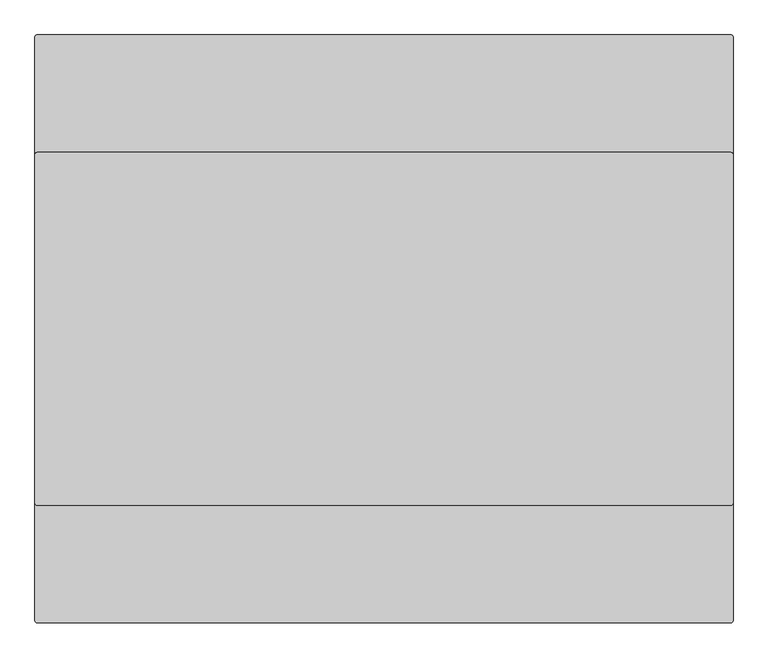
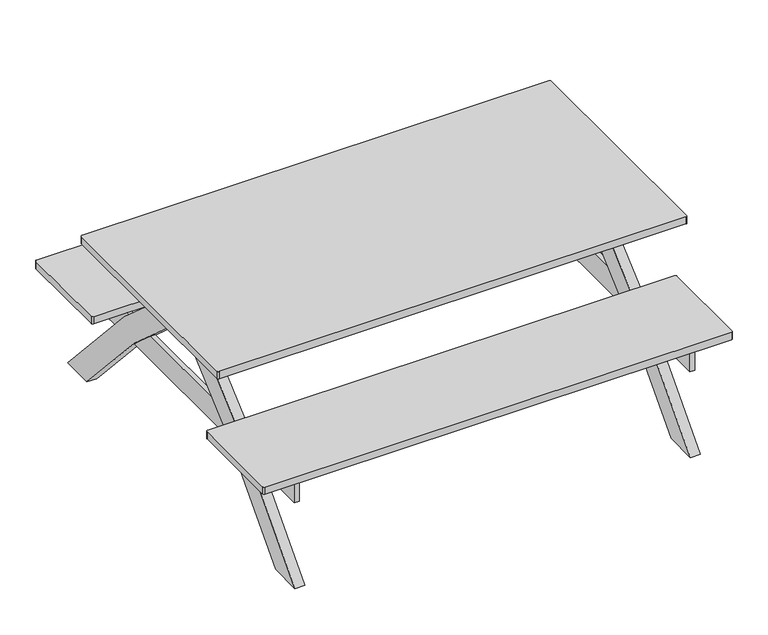
"""IFC4 building model written with IfcOpenShell, lengths in millimetres: furniture geometry, NLRS_90_FU_WPB_picknick tafel_gen_rsf : picknicktafel hout lxbxh 1900x1600x750mm."""

from ifc_helpers import new_model, si_unit, point, frame, frame_2d, origin, place, context, project, spatial, polyline, circle_curve, trimmed, segment, composite_curve, outline, extrude, faceted_brep, source, transform, mapped, element, save


def furniture_9bce7ad1(model_context):
    return source(origin(), model_context, "Body", "SolidModel", [
        extrude(outline(composite_curve([segment(trimmed(circle_curve(frame_2d((943.65, 473.65)), 6.35), [point((943.65, 480.0))], [point((950.0, 473.65))], False, "CARTESIAN"), True, "CONTINUOUS"), segment(polyline([(950.0, 473.65), (950.0, -473.65)]), True, "CONTINUOUS"), segment(trimmed(circle_curve(frame_2d((943.65, -473.65)), 6.35), [point((950.0, -473.65))], [point((943.65, -480.0))], False, "CARTESIAN"), True, "CONTINUOUS"), segment(polyline([(943.65, -480.0), (-943.65, -480.0)]), True, "CONTINUOUS"), segment(trimmed(circle_curve(frame_2d((-943.65, -473.65)), 6.35), [point((-943.65, -480.0))], [point((-950.0, -473.65))], False, "CARTESIAN"), True, "CONTINUOUS"), segment(polyline([(-950.0, -473.65), (-950.0, 473.65)]), True, "CONTINUOUS"), segment(trimmed(circle_curve(frame_2d((-943.65, 473.65)), 6.35), [point((-950.0, 473.65))], [point((-943.65, 480.0))], False, "CARTESIAN"), True, "CONTINUOUS"), segment(polyline([(-943.65, 480.0), (943.65, 480.0)]), True, "CONTINUOUS")], self_intersect=False)), frame((0.0, 0.0, 750.0), z_axis=(0.0, 0.0, 1.0), x_axis=(1.0, 0.0, 0.0)), (0.0, 0.0, 1.0), 30.0),
        extrude(outline(composite_curve([segment(trimmed(circle_curve(frame_2d((943.65, -406.35)), 6.35), [point((943.65, -400.0))], [point((950.0, -406.35))], False, "CARTESIAN"), True, "CONTINUOUS"), segment(polyline([(950.0, -406.35), (950.0, -793.65)]), True, "CONTINUOUS"), segment(trimmed(circle_curve(frame_2d((943.65, -793.65)), 6.35), [point((950.0, -793.65))], [point((943.65, -800.0))], False, "CARTESIAN"), True, "CONTINUOUS"), segment(polyline([(943.65, -800.0), (-943.65, -800.0)]), True, "CONTINUOUS"), segment(trimmed(circle_curve(frame_2d((-943.65, -793.65)), 6.35), [point((-943.65, -800.0))], [point((-950.0, -793.65))], False, "CARTESIAN"), True, "CONTINUOUS"), segment(polyline([(-950.0, -793.65), (-950.0, -406.35)]), True, "CONTINUOUS"), segment(trimmed(circle_curve(frame_2d((-943.65, -406.35)), 6.35), [point((-950.0, -406.35))], [point((-943.65, -400.0))], False, "CARTESIAN"), True, "CONTINUOUS"), segment(polyline([(-943.65, -400.0), (943.65, -400.0)]), True, "CONTINUOUS")], self_intersect=False)), frame((0.0, 0.0, 450.0), z_axis=(0.0, 0.0, 1.0), x_axis=(1.0, 0.0, 0.0)), (0.0, 0.0, 1.0), 30.0),
        extrude(outline(composite_curve([segment(polyline([(943.65, 400.0), (-943.65, 400.0)]), True, "CONTINUOUS"), segment(trimmed(circle_curve(frame_2d((-943.65, 406.35)), 6.35), [point((-943.65, 400.0))], [point((-950.0, 406.35))], False, "CARTESIAN"), True, "CONTINUOUS"), segment(polyline([(-950.0, 406.35), (-950.0, 793.65)]), True, "CONTINUOUS"), segment(trimmed(circle_curve(frame_2d((-943.65, 793.65)), 6.35), [point((-950.0, 793.65))], [point((-943.65, 800.0))], False, "CARTESIAN"), True, "CONTINUOUS"), segment(polyline([(-943.65, 800.0), (943.65, 800.0)]), True, "CONTINUOUS"), segment(trimmed(circle_curve(frame_2d((943.65, 793.65)), 6.35), [point((943.65, 800.0))], [point((950.0, 793.65))], False, "CARTESIAN"), True, "CONTINUOUS"), segment(polyline([(950.0, 793.65), (950.0, 406.35)]), True, "CONTINUOUS"), segment(trimmed(circle_curve(frame_2d((943.65, 406.35)), 6.35), [point((950.0, 406.35))], [point((943.65, 400.0))], False, "CARTESIAN"), True, "CONTINUOUS")], self_intersect=False)), frame((0.0, 0.0, 450.0), z_axis=(0.0, 0.0, 1.0), x_axis=(1.0, 0.0, 0.0)), (0.0, 0.0, 1.0), 30.0),
        extrude(outline(polyline([(-790.0, 774.6), (-790.0, -774.6), (-810.0, -774.6), (-810.0, 774.6), (-790.0, 774.6)])), frame((0.0, 0.0, 350.0), z_axis=(0.0, 0.0, 1.0), x_axis=(1.0, 0.0, 0.0)), (0.0, 0.0, 1.0), 100.0),
        faceted_brep([(780.0, 47.1187461, 750.0), (780.0, 400.0, 437.3), (780.0, 795.7416498, 0.0), (780.0, 660.8726936, 0.0), (780.0, 329.5529767, 366.1128726), (780.0, 1.6260502, 656.7), (780.0, -1.6260502, 656.7), (780.0, -329.5529767, 366.1128726), (780.0, -660.8726936, 0.0), (780.0, -795.7416498, 0.0), (780.0, -400.0, 437.3), (780.0, -47.1187461, 750.0), (820.0, 47.1187461, 750.0), (820.0, -47.1187461, 750.0), (820.0, -400.0, 437.3), (820.0, -795.7416498, 0.0), (820.0, -660.8726936, 0.0), (820.0, -329.5529767, 366.1128726), (820.0, -1.6260502, 656.7), (820.0, 1.6260502, 656.7), (820.0, 329.5529767, 366.1128726), (820.0, 660.8726936, 0.0), (820.0, 795.7416498, 0.0), (820.0, 400.0, 437.3), (810.0, 400.0, 437.3), (810.0, 385.6680783, 450.0), (790.0, 385.6680783, 450.0), (790.0, 400.0, 437.3), (790.0, 479.0035354, 350.0), (810.0, 479.0035354, 350.0), (810.0, 329.5529767, 366.1128726), (810.0, 344.1345792, 350.0), (790.0, 344.1345792, 350.0), (790.0, 329.5529767, 366.1128726), (790.0, 234.8865401, 450.0), (810.0, 234.8865401, 450.0), (810.0, -329.5529767, 366.1128726), (810.0, -234.8865401, 450.0), (790.0, -234.8865401, 450.0), (790.0, -329.5529767, 366.1128726), (790.0, -344.1345792, 350.0), (810.0, -344.1345792, 350.0), (810.0, -400.0, 437.3), (810.0, -479.0035354, 350.0), (790.0, -479.0035354, 350.0), (790.0, -400.0, 437.3), (790.0, -385.6680783, 450.0), (810.0, -385.6680783, 450.0), (790.0, 774.6, 450.0), (790.0, 774.6, 350.0), (790.0, -774.6, 350.0), (790.0, -774.6, 450.0), (810.0, -774.6, 450.0), (810.0, -774.6, 350.0), (810.0, 774.6, 350.0), (810.0, 774.6, 450.0)], [[[0, 1, 2, 3, 4, 5, 6, 7, 8, 9, 10, 11]], [[12, 13, 14, 15, 16, 17, 18, 19, 20, 21, 22, 23]], [[1, 0, 12, 23, 24, 25, 26, 27]], [[2, 1, 27, 28, 29, 24, 23, 22]], [[3, 2, 22, 21]], [[4, 3, 21, 20, 30, 31, 32, 33]], [[5, 4, 33, 34, 35, 30, 20, 19]], [[6, 5, 19, 18]], [[7, 6, 18, 17, 36, 37, 38, 39]], [[8, 7, 39, 40, 41, 36, 17, 16]], [[9, 8, 16, 15]], [[10, 9, 15, 14, 42, 43, 44, 45]], [[11, 10, 45, 46, 47, 42, 14, 13]], [[0, 11, 13, 12]], [[48, 49, 28, 27, 26]], [[50, 51, 46, 45, 44]], [[38, 34, 33, 32, 40, 39]], [[52, 53, 43, 42, 47]], [[54, 55, 25, 24, 29]], [[41, 31, 30, 35, 37, 36]], [[37, 35, 34, 38]], [[51, 52, 47, 46]], [[55, 48, 26, 25]], [[49, 48, 55, 54]], [[31, 41, 40, 32]], [[49, 54, 29, 28]], [[53, 50, 44, 43]], [[51, 50, 53, 52]]]),
        extrude(outline(polyline([(47.1187461, 750.0), (400.0, 437.3), (795.7416498, 0.0), (660.8726936, 0.0), (329.5529767, 366.1128726), (1.6260502, 656.7), (-1.6260502, 656.7), (-329.5529767, 366.1128726), (-660.8726936, 0.0), (-795.7416498, 0.0), (-400.0, 437.3), (-47.1187461, 750.0), (47.1187461, 750.0)])), frame((-820.0, 0.0, 0.0), z_axis=(1.0, 0.0, 0.0), x_axis=(0.0, 1.0, 0.0)), (0.0, 0.0, 1.0), 40.0),
    ])


if __name__ == "__main__":
    model = new_model("IFC4")
    model_context = context("Model", 3, world=origin())
    ifc_project = project(units=[si_unit("LENGTHUNIT", "METRE", prefix="MILLI")], contexts=[model_context])
    site = spatial("IfcSite", under=ifc_project)
    building = spatial("IfcBuilding", under=site)
    placement = place(None, origin())
    furniture_shape = furniture_9bce7ad1(model_context)
    element("IfcFurniture", 1, ObjectType="NLRS_90_FU_WPB_picknick tafel_gen_rsf : picknicktafel hout lxbxh 1900x1600x750mm", at=placement, inside=building, context=model_context, shape_type="MappedRepresentation", body=[
        mapped(furniture_shape, transform((0.0, 0.0, 0.0), x_axis=(1.0, 0.0, 0.0), y_axis=(0.0, 1.0, 0.0), z_axis=(0.0, 0.0, 1.0))),
    ])
    save(model, "model.ifc")

# Revit data of these elements
# Type "NLRS_90_FU_WPB_picknick tafel_gen_rsf : picknicktafel hout lxbxh 1900x1600x750mm"
#   Type IFC Predefined Type = "USERDEFINED"
#   Export Type to IFC As = "IfcGeographicElementType"
#   Type IfcGUID = "05J6pyYiTDtR2exmlhyPT4"
#   IfcName[Type] = "picknicktafel hout lxbxh 1900x1600x750mm"
#   IfcDescription[Type] = "picknicktafel hout lxbxh 1900x1600x750mm"
#   IfcObjectType[Type] = "TABLE"
#   IfcExportAs[Type] = "IfcGeographicElementType"
#   IfcExportType[Type] = "USERDEFINED"
#   NLRS_C_omschrijving_02 [instance default] = "zitbank"
#   NLRS_C_omschrijving_01 [instance default] = "tafelblad"
#   NLRS_C_revit_versie = ""
#   NLRS_C_content_versie = ""
#   NLRS_C_content_provider = ""
#   NLRS_C_content_handleiding = ""
#   NLRS_C_content_datum_uitgifte = ""
#   NLRS_C_content_datum_gewijzigd = ""
#   NLRS_C_content_creator = ""
#   Model = "generiek"
#   Manufacturer = "Revit Standards Foundation"
#   Description = "picknicktafel hout lxbxh 1900x1600x750mm"
#   Assembly Code = "90.71"
#   bf_overstek = 150.00 mm
#   NLRS_C_hoogte_01 = 450.00 mm
#   NLRS_C_hoogte = 750.00 mm
#   NLRS_C_dikte_02 = 30.00 mm
#   NLRS_C_dikte_01 = 30.00 mm
#   NLRS_C_diepte_02 = 960.00 mm
#   NLRS_C_diepte_01 = 400.00 mm
#   NLRS_C_diepte = 1600.00 mm
#   NLRS_C_breedte = 1900.00 mm
#   Default Elevation = 1219.20 mm
#   NLRS_C_materiaal_02 = NLRS_i3_hout loofhout meranti vernis planken 120mm_gen_rsf
#   NLRS_C_materiaal_01 = NLRS_i3_hout loofhout meranti vernis planken 120mm_gen_rsf
#   NLRS_C_materiaal = NLRS_i3_hout loofhout meranti vernis_gen_rsf
# Element 1 (IfcFurniture, "NLRS_90_FU_WPB_picknick tafel_gen_rsf : picknicktafel hout lxbxh 1900x1600x750mm")
#   Materials on its faces: "NLRS_i3_hout loofhout meranti vernis_gen_rsf", "NLRS_i3_hout loofhout meranti vernis planken 120mm_gen_rsf"
# Materials
#   "NLRS_i3_hout loofhout meranti vernis planken 120mm_gen_rsf": class "Unassigned", colour RGB 227 170 128, transparency 0, Keynote = "i3", Model = "generiek", Manufacturer = "Revit Standards Foundation", URL = "www.revitstandards.org", Description = "loofhout merantie vernis planken 120mm", Cost = 0
#   "NLRS_i3_hout loofhout meranti vernis_gen_rsf": class "Unassigned", colour RGB 227 170 128, transparency 0, Keynote = "i3", Model = "generiek", Manufacturer = "Revit Standards Foundation", URL = "www.revitstandards.org", Description = "loofhout merantie vernis", Cost = 0
